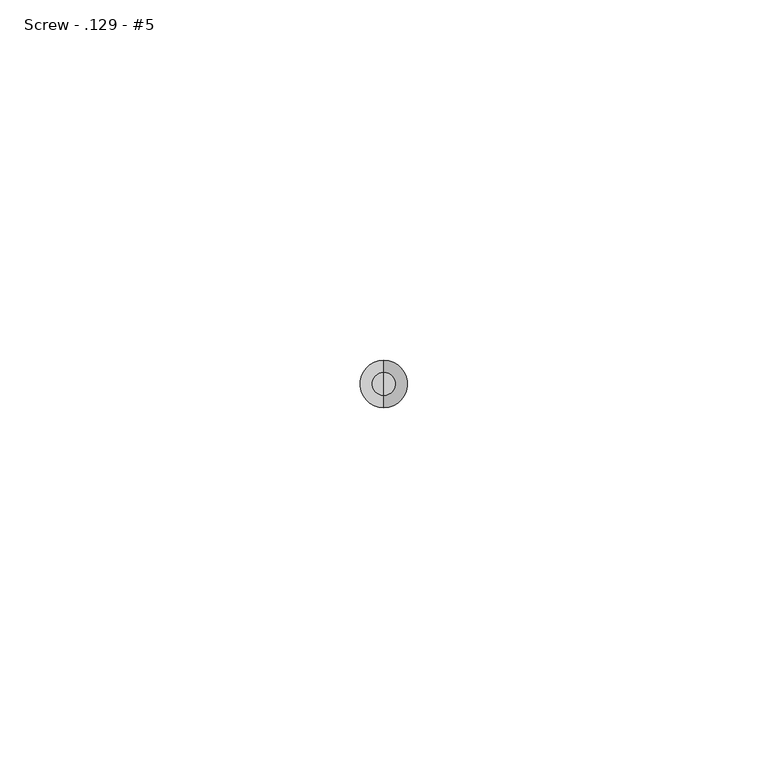
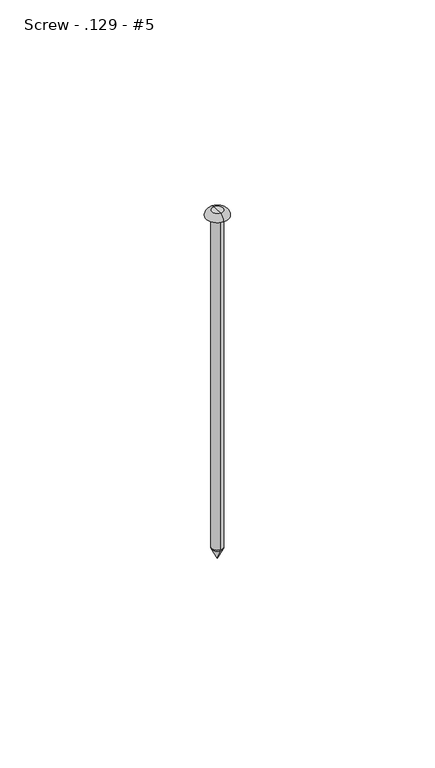
"""IFC4 building model written with IfcOpenShell, lengths in millimetres: fastener geometry, 060523 - W_P_C - Fastenings - Generic : Screw - .129 - #5."""

from ifc_helpers import new_model, si_unit, point, frame, origin, origin_2d, place, context, project, spatial, polyline, circle_curve, ellipse_curve, trimmed, segment, composite_curve, outline, extrude, source, transform, mapped, element, save
from ifc_brep_helpers import plane_surface, revolved_surface, advanced_brep


def screw_129_5_ee0959b3(model_context):
    return source(origin(), model_context, "Body", "SolidModel", [
        advanced_brep(
        [(0.0, -1.6383, -101.6), (0.0, 1.6383, -101.6), (0.0, 0.0, -101.6), (0.0, 0.0, -104.8766)],
        [
            (0, 1, circle_curve(frame((0.0, 0.0, -101.6), z_axis=(0.0, 0.0, 1.0), x_axis=(0.0, 1.0, 0.0)), 1.6383)),
            (1, 2),
            (2, 0),
            (1, 0, circle_curve(frame((0.0, 0.0, -101.6), z_axis=(0.0, 0.0, 1.0), x_axis=(0.0, 1.0, 0.0)), 1.6383)),
            (3, 1),
            (0, 3),
        ],
        [
            plane_surface(frame((0.0, 0.0, -101.6), z_axis=(0.0, 0.0, 1.0), x_axis=(0.0, 1.0, 0.0))),
            revolved_surface(polyline([(0.0, 1.6383, -101.6), (0.0, 0.0, -104.8766)]), (0.0, 0.0, -103.0840259), (0.0, 0.0, -1.0)),
        ],
        [
            (0, [[1, 2, 3]]),
            (0, [[4, -3, -2]]),
            (1, [[5, -1, 6]]),
            (1, [[-6, -4, -5]]),
        ],
    ),
        advanced_brep(
        [(0.0, 3.2766, 0.0), (0.0, -3.2766, 0.0), (0.0, 0.0, 0.0), (0.0, 0.0, 1.6383), (0.0, -1.5875, 1.6383), (0.0, 1.5875, 1.6383)],
        [
            (0, 1, circle_curve(frame((0.0, 0.0, 0.0), z_axis=(0.0, 0.0, -1.0), x_axis=(0.0, -1.0, 0.0)), 3.2766)),
            (1, 2),
            (2, 0),
            (1, 0, circle_curve(frame((0.0, 0.0, 0.0), z_axis=(0.0, 0.0, -1.0), x_axis=(0.0, -1.0, 0.0)), 3.2766)),
            (3, 4),
            (4, 5, circle_curve(frame((0.0, 0.0, 1.6383), z_axis=(0.0, 0.0, 1.0), x_axis=(0.0, -1.0, 0.0)), 1.5875)),
            (5, 3),
            (5, 4, circle_curve(frame((0.0, 0.0, 1.6383), z_axis=(0.0, 0.0, 1.0), x_axis=(0.0, -1.0, 0.0)), 1.5875)),
            (4, 1, circle_curve(frame((0.0, -1.5875, -0.0515876), z_axis=(1.0, 0.0, 0.0), x_axis=(0.0, -1.0, 0.0)), 1.6898876)),
            (0, 5, circle_curve(frame((0.0, 1.5875, -0.0515876), z_axis=(1.0, 0.0, 0.0), x_axis=(0.0, 1.0, 0.0)), 1.6898876)),
        ],
        [
            plane_surface(frame((0.0, 0.0, 0.0), z_axis=(0.0, 0.0, -1.0), x_axis=(0.0, -1.0, 0.0))),
            plane_surface(frame((0.0, 0.0, 1.6383), z_axis=(0.0, 0.0, 1.0), x_axis=(0.0, -1.0, 0.0))),
            revolved_surface(trimmed(ellipse_curve(frame((0.0, -1.5875, -0.0515876), z_axis=(-1.0, 0.0, 0.0), x_axis=(0.0, -1.0, 0.0)), 1.6898876, 1.6898876), [point((0.0, -3.2766, 0.0))], [point((0.0, -1.5875, 1.6383))], True, "CARTESIAN"), (0.0, 0.0, 1.4840259), (0.0, 0.0, 1.0)),
        ],
        [
            (0, [[1, 2, 3]]),
            (0, [[4, -3, -2]]),
            (1, [[5, 6, 7]]),
            (1, [[-7, 8, -5]]),
            (2, [[-6, 9, -1, 10]]),
            (2, [[-8, -10, -4, -9]]),
        ],
    ),
        extrude(outline(composite_curve([segment(trimmed(circle_curve(origin_2d(), 1.6383), [point((0.0, -1.6383))], [point((0.0, 1.6383))], False, "CARTESIAN"), True, "CONTINUOUS"), segment(trimmed(circle_curve(origin_2d(), 1.6383), [point((0.0, 1.6383))], [point((0.0, -1.6383))], False, "CARTESIAN"), True, "CONTINUOUS")], self_intersect=False)), frame((0.0, 0.0, -101.6), z_axis=(0.0, 0.0, 1.0), x_axis=(1.0, 0.0, 0.0)), (0.0, 0.0, 1.0), 101.6),
    ])


if __name__ == "__main__":
    model = new_model("IFC4")
    model_context = context("Model", 3, world=origin())
    ifc_project = project(units=[si_unit("LENGTHUNIT", "METRE", prefix="MILLI")], contexts=[model_context])
    site = spatial("IfcSite", under=ifc_project)
    building = spatial("IfcBuilding", under=site)
    placement = place(None, origin())
    screw_129_5_shape = screw_129_5_ee0959b3(model_context)
    element("IfcFastener", 1, ObjectType="060523 - W_P_C - Fastenings - Generic : Screw - .129 - #5", at=placement, inside=building, context=model_context, shape_type="MappedRepresentation", body=[
        mapped(screw_129_5_shape, transform((0.0, 0.0, 0.0), x_axis=(1.0, 0.0, 0.0), y_axis=(0.0, 1.0, 0.0), z_axis=(0.0, 0.0, 1.0))),
    ])
    save(model, "model.ifc")

# Revit data of these elements
# Type "060523 - W_P_C - Fastenings - Generic : Screw - .129 - #5"
#   Washer_Thickness = 0' - 0.00333"
#   Washer Radius = 0' - 0.0745"
#   Washer Offset - Head = 0' - 0"
#   Washer Offset = 0' - 0"
#   Thickness_of_Substrate [instance default] = 0' - 1"
#   Side = 0' - 0 37/64"
#   Radius = 0' - 0.0645"
#   Length [instance default] = 0' - 4"
#   Head Size = 0' - 1"
#   Head Radius = 0' - 0 1/2"
#   Head Height = 0' - 0.01"
#   Double Diameter = 0' - 0.258"
#   Diameter = 0' - 0.129"
#   Default Elevation = 4' - 0"
#   Washer_Nut_Visibility = no
#   Washer_Head_Visibility = no
#   Round_Head_Visibility = yes
#   Point Visibility = yes
#   Nut_Visibility = no
#   Hex_Head_Visiblilty = no
#   Washer Material = none
#   Bolt Material (Size) = AT SILL - FASTENER AT 24" O.C.
# Element 1 (IfcFastener, "060523 - W_P_C - Fastenings - Generic : Screw - .129 - #5")
#   Materials on its faces: "AT SILL - FASTENER AT 24\" O.C."
# Materials
#   "AT SILL - FASTENER AT 24\" O.C.": class "Generic", colour RGB 120 120 120, transparency 0, Cost = 0
